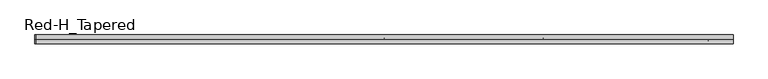
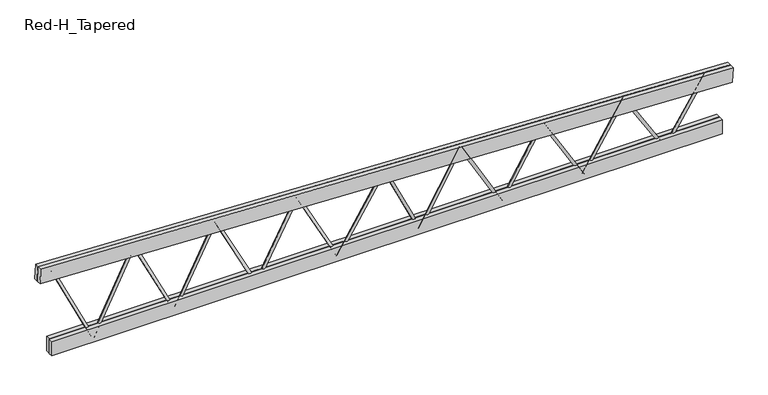
"""IFC4 building model written with IfcOpenShell, lengths in millimetres: beam geometry, Construction_Frames_RedBuilt_Openweb_Red-H_Tapered : Red-H_Tapered."""

from ifc_helpers import new_model, si_unit, point, frame, origin, origin_2d, place, context, project, spatial, polyline, circle_curve, trimmed, segment, composite_curve, outline, extrude, source, transform, mapped, element, save


def red_h_tapered_ff799f4f(model_context):
    return source(origin(), model_context, "Body", "SweptSolid", [
        extrude(outline(composite_curve([segment(trimmed(circle_curve(origin_2d(), 12.7), [point((0.0, 12.7))], [point((0.0, -12.7))], False, "CARTESIAN"), True, "CONTINUOUS"), segment(trimmed(circle_curve(origin_2d(), 12.7), [point((0.0, -12.7))], [point((0.0, 12.7))], False, "CARTESIAN"), True, "CONTINUOUS")], self_intersect=False)), frame((2576.1482728, 0.0, -367.0101562), z_axis=(0.5404734297056486, 0.0, 0.8413610828783403), x_axis=(0.0, -1.0, 0.0)), (0.0, 0.0, 1.0), 694.3511079),
        extrude(outline(composite_curve([segment(trimmed(circle_curve(origin_2d(), 12.7), [point((0.0, -12.7000001))], [point((0.0, 12.7))], False, "CARTESIAN"), True, "CONTINUOUS"), segment(trimmed(circle_curve(origin_2d(), 12.7), [point((0.0, 12.7))], [point((0.0, -12.7000001))], False, "CARTESIAN"), True, "CONTINUOUS")], self_intersect=False)), frame((2576.1482728, 0.0, -367.0101562), z_axis=(-0.5247393086940249, 0.0, 0.8512629781162322), x_axis=(0.0, -1.0, 0.0)), (0.0, 0.0, 1.0), 715.1709782),
        extrude(outline(composite_curve([segment(trimmed(circle_curve(origin_2d(), 12.7), [point((0.0, 12.7))], [point((0.0, -12.7))], False, "CARTESIAN"), True, "CONTINUOUS"), segment(trimmed(circle_curve(origin_2d(), 12.7), [point((0.0, -12.7))], [point((0.0, 12.7))], False, "CARTESIAN"), True, "CONTINUOUS")], self_intersect=False)), frame((1825.5916234, 0.0, -367.0101562), z_axis=(0.5247393086940241, 0.0, 0.8512629781162327), x_axis=(0.0, -1.0, 0.0)), (0.0, 0.0, 1.0), 715.1709782),
        extrude(outline(composite_curve([segment(trimmed(circle_curve(origin_2d(), 12.7), [point((0.0, -12.7))], [point((0.0, 12.6999999))], False, "CARTESIAN"), True, "CONTINUOUS"), segment(trimmed(circle_curve(origin_2d(), 12.7), [point((0.0, 12.6999999))], [point((0.0, -12.7))], False, "CARTESIAN"), True, "CONTINUOUS")], self_intersect=False)), frame((1825.5916234, 0.0, -367.0101562), z_axis=(-0.5097338931901324, 0.0, 0.860332120830805), x_axis=(0.0, -1.0, 0.0)), (0.0, 0.0, 1.0), 736.2239978),
        extrude(outline(composite_curve([segment(trimmed(circle_curve(origin_2d(), 12.7), [point((0.0, 12.7000001))], [point((0.0, -12.6999999))], False, "CARTESIAN"), True, "CONTINUOUS"), segment(trimmed(circle_curve(origin_2d(), 12.7), [point((0.0, -12.6999999))], [point((0.0, 12.7000001))], False, "CARTESIAN"), True, "CONTINUOUS")], self_intersect=False)), frame((1075.034974, 0.0, -367.0101562), z_axis=(0.5097338931901313, 0.0, 0.8603321208308056), x_axis=(0.0, -1.0, 0.0)), (0.0, 0.0, 1.0), 736.2239978),
        extrude(outline(composite_curve([segment(trimmed(circle_curve(origin_2d(), 12.7), [point((0.0, -12.7))], [point((0.0, 12.7))], False, "CARTESIAN"), True, "CONTINUOUS"), segment(trimmed(circle_curve(origin_2d(), 12.7), [point((0.0, 12.7))], [point((0.0, -12.7))], False, "CARTESIAN"), True, "CONTINUOUS")], self_intersect=False)), frame((1075.034974, 0.0, -367.0101562), z_axis=(-0.4954229948377255, 0.0, 0.8686518613265151), x_axis=(0.0, -1.0, 0.0)), (0.0, 0.0, 1.0), 757.4907273),
        extrude(outline(composite_curve([segment(trimmed(circle_curve(origin_2d(), 12.7), [point((0.0, 12.7))], [point((0.0, -12.7))], False, "CARTESIAN"), True, "CONTINUOUS"), segment(trimmed(circle_curve(origin_2d(), 12.7), [point((0.0, -12.7))], [point((0.0, 12.7))], False, "CARTESIAN"), True, "CONTINUOUS")], self_intersect=False)), frame((324.4783247, 0.0, -367.0101562), z_axis=(0.495422994837726, 0.0, 0.8686518613265147), x_axis=(0.0, -1.0, 0.0)), (0.0, 0.0, 1.0), 757.4907273),
        extrude(outline(composite_curve([segment(trimmed(circle_curve(origin_2d(), 12.7), [point((0.0, -12.7000001))], [point((0.0, 12.7))], False, "CARTESIAN"), True, "CONTINUOUS"), segment(trimmed(circle_curve(origin_2d(), 12.7), [point((0.0, 12.7))], [point((0.0, -12.7000001))], False, "CARTESIAN"), True, "CONTINUOUS")], self_intersect=False)), frame((324.4783247, 0.0, -367.0101562), z_axis=(-0.4293223949598947, 0.0, 0.9031513058097742), x_axis=(0.0, -1.0, 0.0)), (0.0, 0.0, 1.0), 755.7917511),
        extrude(outline(composite_curve([segment(trimmed(circle_curve(origin_2d(), 12.7), [point((0.0, -12.7))], [point((0.0, 12.7))], False, "CARTESIAN"), True, "CONTINUOUS"), segment(trimmed(circle_curve(origin_2d(), 12.7), [point((0.0, 12.7))], [point((0.0, -12.7))], False, "CARTESIAN"), True, "CONTINUOUS")], self_intersect=False)), frame((-426.0783247, 0.0, -367.0101562), z_axis=(0.5295134852617149, 0.0, 0.8483015200540381), x_axis=(0.0, -1.0, 0.0)), (0.0, 0.0, 1.0), 804.6600069),
        extrude(outline(composite_curve([segment(trimmed(circle_curve(origin_2d(), 12.7), [point((0.0, 12.7))], [point((0.0, -12.7))], False, "CARTESIAN"), True, "CONTINUOUS"), segment(trimmed(circle_curve(origin_2d(), 12.7), [point((0.0, -12.7))], [point((0.0, 12.7))], False, "CARTESIAN"), True, "CONTINUOUS")], self_intersect=False)), frame((-426.0783247, 0.0, -367.0101562), z_axis=(-0.4687480882122886, 0.0, 0.8833318910790692), x_axis=(0.0, -1.0, 0.0)), (0.0, 0.0, 1.0), 800.5970245),
        extrude(outline(composite_curve([segment(trimmed(circle_curve(origin_2d(), 12.7), [point((0.0, -12.7000001))], [point((0.0, 12.7))], False, "CARTESIAN"), True, "CONTINUOUS"), segment(trimmed(circle_curve(origin_2d(), 12.7), [point((0.0, 12.7))], [point((0.0, -12.7000001))], False, "CARTESIAN"), True, "CONTINUOUS")], self_intersect=False)), frame((-1176.634974, 0.0, -367.0101562), z_axis=(0.4687480882122872, 0.0, 0.88333189107907), x_axis=(0.0, -1.0, 0.0)), (0.0, 0.0, 1.0), 800.5970245),
        extrude(outline(composite_curve([segment(trimmed(circle_curve(origin_2d(), 12.7), [point((0.0, 12.6999999))], [point((0.0, -12.7000001))], False, "CARTESIAN"), True, "CONTINUOUS"), segment(trimmed(circle_curve(origin_2d(), 12.7), [point((0.0, -12.7000001))], [point((0.0, 12.6999999))], False, "CARTESIAN"), True, "CONTINUOUS")], self_intersect=False)), frame((-1176.634974, 0.0, -367.0101562), z_axis=(-0.45631727596060173, 0.0, 0.8898171405743408), x_axis=(0.0, -1.0, 0.0)), (0.0, 0.0, 1.0), 822.4065676),
        extrude(outline(composite_curve([segment(trimmed(circle_curve(origin_2d(), 12.7), [point((0.0, -12.7))], [point((0.0, 12.7000001))], False, "CARTESIAN"), True, "CONTINUOUS"), segment(trimmed(circle_curve(origin_2d(), 12.7), [point((0.0, 12.7000001))], [point((0.0, -12.7))], False, "CARTESIAN"), True, "CONTINUOUS")], self_intersect=False)), frame((-1927.1916234, 0.0, -367.0101562), z_axis=(0.45631727596061405, 0.0, 0.8898171405743345), x_axis=(0.0, -1.0, 0.0)), (0.0, 0.0, 1.0), 822.4065676),
        extrude(outline(composite_curve([segment(trimmed(circle_curve(origin_2d(), 12.7), [point((0.0, 12.7))], [point((0.0, -12.7000001))], False, "CARTESIAN"), True, "CONTINUOUS"), segment(trimmed(circle_curve(origin_2d(), 12.7), [point((0.0, -12.7000001))], [point((0.0, 12.7))], False, "CARTESIAN"), True, "CONTINUOUS")], self_intersect=False)), frame((-1927.1916234, 0.0, -367.0101562), z_axis=(-0.44444803179616443, 0.0, 0.8958046366437917), x_axis=(0.0, -1.0, 0.0)), (0.0, 0.0, 1.0), 844.3694152),
        extrude(outline(composite_curve([segment(trimmed(circle_curve(origin_2d(), 12.7), [point((0.0, -12.6999999))], [point((0.0, 12.7000001))], False, "CARTESIAN"), True, "CONTINUOUS"), segment(trimmed(circle_curve(origin_2d(), 12.7), [point((0.0, 12.7000001))], [point((0.0, -12.6999999))], False, "CARTESIAN"), True, "CONTINUOUS")], self_intersect=False)), frame((-2677.7482728, 0.0, -367.0101562), z_axis=(0.4444480317961537, 0.0, 0.8958046366437971), x_axis=(0.0, -1.0, 0.0)), (0.0, 0.0, 1.0), 844.3694152),
        extrude(outline(composite_curve([segment(trimmed(circle_curve(origin_2d(), 12.7), [point((0.0, 12.7))], [point((0.0, -12.7))], False, "CARTESIAN"), True, "CONTINUOUS"), segment(trimmed(circle_curve(origin_2d(), 12.7), [point((0.0, -12.7))], [point((0.0, 12.7))], False, "CARTESIAN"), True, "CONTINUOUS")], self_intersect=False)), frame((-2677.7482728, 0.0, -367.0101562), z_axis=(-0.43310978037460907, 0.0, 0.9013411774371889), x_axis=(0.0, -1.0, 0.0)), (0.0, 0.0, 1.0), 866.4739096),
        extrude(outline(polyline([(-3078.4265974, -41.275), (-3078.4265974, -3.175), (3078.4265974, -3.175), (3078.4265974, -41.275), (-3078.4265974, -41.275)])), frame((0.0, 0.0, -386.0601562), z_axis=(0.0, 0.0, 1.0), x_axis=(1.0, 0.0, 0.0)), (0.0, 0.0, 1.0), 139.7),
        extrude(outline(polyline([(-3078.4265974, 3.175), (-3078.4265974, 41.275), (3078.4265974, 41.275), (3078.4265974, 3.175), (-3078.4265974, 3.175)])), frame((0.0, 0.0, -386.0601562), z_axis=(0.0, 0.0, 1.0), x_axis=(1.0, 0.0, 0.0)), (0.0, 0.0, 1.0), 139.7),
        extrude(outline(polyline([(0.0, -38.1), (0.0, 0.0), (6365.6425859, 0.0), (6365.6425859, -38.1), (0.0, -38.1)])), frame((-3185.8795792, -3.175, 350.6625082), z_axis=(0.041896791470728445, 0.0, 0.9991219439410078), x_axis=(0.9991219439410078, 0.0, -0.041896791470728445)), (0.0, 0.0, 1.0), 139.7),
        extrude(outline(polyline([(0.0, -38.1), (0.0, 0.0), (6365.6425859, 0.0), (6365.6425859, -38.1), (0.0, -38.1)])), frame((-3185.8795792, 41.275, 350.6625082), z_axis=(0.04189679147072844, 0.0, 0.9991219439410078), x_axis=(0.9991219439410078, 0.0, -0.04189679147072844)), (0.0, 0.0, 1.0), 139.7),
    ])


if __name__ == "__main__":
    model = new_model("IFC4")
    model_context = context("Model", 3, world=origin())
    ifc_project = project(units=[si_unit("LENGTHUNIT", "METRE", prefix="MILLI")], contexts=[model_context])
    site = spatial("IfcSite", under=ifc_project)
    building = spatial("IfcBuilding", under=site)
    placement = place(None, origin())
    red_h_tapered_shape = red_h_tapered_ff799f4f(model_context)
    element("IfcBeam", 1, ObjectType="Construction_Frames_RedBuilt_Openweb_Red-H_Tapered : Red-H_Tapered", at=placement, inside=building, context=model_context, shape_type="MappedRepresentation", body=[
        mapped(red_h_tapered_shape, transform((0.0, 0.0, 0.0), x_axis=(1.0, 0.0, 0.0), y_axis=(0.0, 1.0, 0.0), z_axis=(0.0, 0.0, 1.0))),
    ])
    save(model, "model.ifc")

# Revit data of these elements
# Type "Construction_Frames_RedBuilt_Openweb_Red-H_Tapered : Red-H_Tapered"
#   Youtube clip = ""
#   Weight Net (Kg) = "0"
#   Webs = "Up to 2\" diameter tubular steel"
#   Uniformat II Description = ""
#   Uniformat II Code = ""
#   Uniclass 2015 Name = "Softwood trusses"
#   Uniclass 2015 Code = "Pr_20_85_90_81"
#   Uniclass 2.0 Description = "Structural Framing Systems"
#   Uniclass 2.0 Code = "SS-15-10-75"
#   Uniclass 1.4 Description = "Trusses"
#   Uniclass 1.4 Code = "L3523"
#   UNSPSC Code = "30103606"
#   Technical description = "http://www.redbuilt.com/reference/literature-and-other-resources"
#   Region South America = "None"
#   Region Oceania = "None"
#   Region North America = "US"
#   Region Middle East = "None"
#   Region Europe = "None"
#   Region Asia = "None"
#   Region Antarctica = "None"
#   Region Africa = "None"
#   QR code = "http://bimobject.com/redbuilt/product/redbuilt-0003"
#   Product url = "http://www.redbuilt.com/products/default.aspx?id=2"
#   Product group = "Wood Trusses"
#   Product family = "Construction"
#   Product data url = "https://bimobject.com/redbuilt/product/redbuilt-0003"
#   Product certification = ""
#   Product SKU = "redbuilt-0003"
#   Product Page URL = "http://www.redbuilt.com/commercial-systems/red-m-red-h-open-web-trusses"
#   Product Guid = "2c5793f2-6ffb-4665-b825-cf90c048e711"
#   Product Documentation Link = "http://www.redbuilt.com/documents/OW_Guide_2017_07_LowRes_wLinks.pdf"
#   OmniClass Description = "Wood Trusses"
#   OmniClass Code = "23-13 35 19 13 17"
#   NBS Reference Description = ""
#   NBS Reference Code = ""
#   Material secondary = "Steel"
#   Material main = "CHARRED WOOD"
#   Masterformat 2014 Description = "Metal-Web Wood Joists"
#   Masterformat 2014 Code = "06 17 36"
#   Manufacturer name = "RedBuilt"
#   Manufacturer country = "United States"
#   Installation instructions = "http://www.redbuilt.com/documents/Installation_Sheets_Open-Web.pdf"
#   IFC Classification = ""
#   EAN code = ""
#   Design country = "United States"
#   Product Information = "http://redbuilt.com/products/default.aspx?id=2"
#   Model = "Red-H-Tapered"
#   Manufacturer URL = "http://redbuilt.com/"
#   Manufacturer = "RedBuilt™"
#   Description = "Open Web Truss"
#   Date of publishing = "8/17/2010"
#   Contact us = "http://redbuilt.com/contact/"
#   Chords = "Double 1½\" x 5½\" MSR lumber"
#   COBIe Type Category = ""
#   Brand url = "http://www.redbuilt.com"
#   BIMobject main category code = "construction"
#   BIMobject main category = "Construction"
#   BIMobject category code = "construction-frames-trusses"
#   BIMobject category = "Frames & Trusses"
#   Web Radius = 0' - 0 1/2"
#   Web Layout Offset Start [instance default] = 0' - 5"
#   Web Layout Offset End [instance default] = 0' - 5"
#   Web Diameter = 0' - 1"
#   TotalLength [instance default] = 20' - 0"
#   Span Minimum = 4' - 0"
#   Span Maximum = 70' - 0"
#   Span Limit [instance default] = 20' - 0"
#   Nominal width = 0' - 0"
#   Nominal height = 0' - 0"
#   Inner Depth Top [instance default] = 0' - 2.76372"
#   Depth Start [instance default] = 6' - 0"
#   Top Chord Length [instance default] = 20' - 1.19701"
#   TC Extension Start Aux [instance default] = 0' - 0"
#   TC Extension End Aux [instance default] = 0' - 0"
#   T-B Chord Length Difference L [instance default] = 0' - 4"
#   T-B Chord Length Difference [instance default] = 0' - 4"
#   Height 2 [instance default] = 6' - 0"
#   Depth Minimum at Wall = 2' - 0"
#   Depth Maximum at Wall = 6' - 0"
#   Depth Lower End [instance default] = 2' - 0"
#   Depth Higher End [instance default] = 6' - 0"
#   Depth End [instance default] = 2' - 0"
#   Depth 2 [instance default] = 2' - 0"
#   Chord Width = 0' - 3 1/4"
#   Chord Thickness = 0' - 1 1/2"
#   Chord Depth = 0' - 5 1/2"
#   Offset Start [instance default] = 0' - 0"
#   TC Extension Start [instance default] = 0' - 0"
#   End Panel = 0' - 5"
#   Offset End [instance default] = 0' - 0"
#   TC Extension End [instance default] = 0' - 0"
#   Length [instance default] = 20' - 0"
#   Angle [instance default] = 5.71059°
#   Span Limit Warning [instance default] = no
#   Edition number = 1
#   Top Bearing Start [instance default] = yes
#   Top Bearing End [instance default] = yes
#   Bottom Bearing Start [instance default] = no
#   Bottom Bearing End [instance default] = no
#   8 Panels [instance default] = yes
#   16 Panels [instance default] = no
#   12 Panels [instance default] = no
#   Web Material = RedBuilt-Steel, Galvanized
#   Clip Material = RedBuilt-Steel, Galvanized
#   Chords Material = OPEN WEB TRUSSES - WOOD TOP/BOTTOM CHORD - TUBE STEEL WEBS
#   URL = ""
#   Assembly Code = ""
# Element 1 (IfcBeam, "Construction_Frames_RedBuilt_Openweb_Red-H_Tapered : Red-H_Tapered")
#   Web Layout Offset End = 0' - 9"
#   TotalLength = 20' - 10.3958"
#   Span Limit = 20' - 10.3958"
#   Inner Depth Top = 0' - 2.75242"
#   Depth Start = 0' - 0"
#   Top Chord Length = 20' - 10.61585"
#   TC Extension End Aux = 0' - 4"
#   Height 2 = 0' - 0"
#   Depth Higher End = 0' - 0"
#   Depth 2 = 0' - 10 1/2"
#   Offset End = 0' - 4"
#   Angle = 2.40121°
#   Materials on its faces: "RedBuilt-Steel, Galvanized", "OPEN WEB TRUSSES - WOOD TOP/BOTTOM CHORD - TUBE STEEL WEBS"
# Materials
#   "RedBuilt-Steel, Galvanized": class "Metal", colour RGB 164 172 176, transparency 0, Manufacturer = "RedBuilt. LLC", Comments = "Openweb Metal Web", URL = "http://www.redbuilt.com/", Description = "Galvanized steel", Cost = 0
#   "OPEN WEB TRUSSES - WOOD TOP/BOTTOM CHORD - TUBE STEEL WEBS": class "Wood", colour RGB 198 202 183, transparency 0, Description = "Generic wood", Cost = 0
